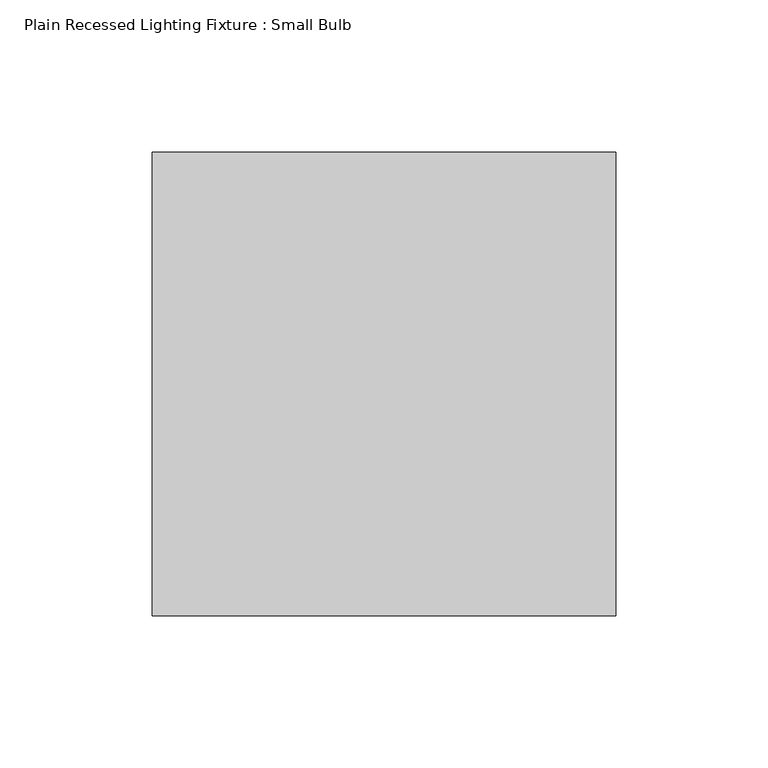
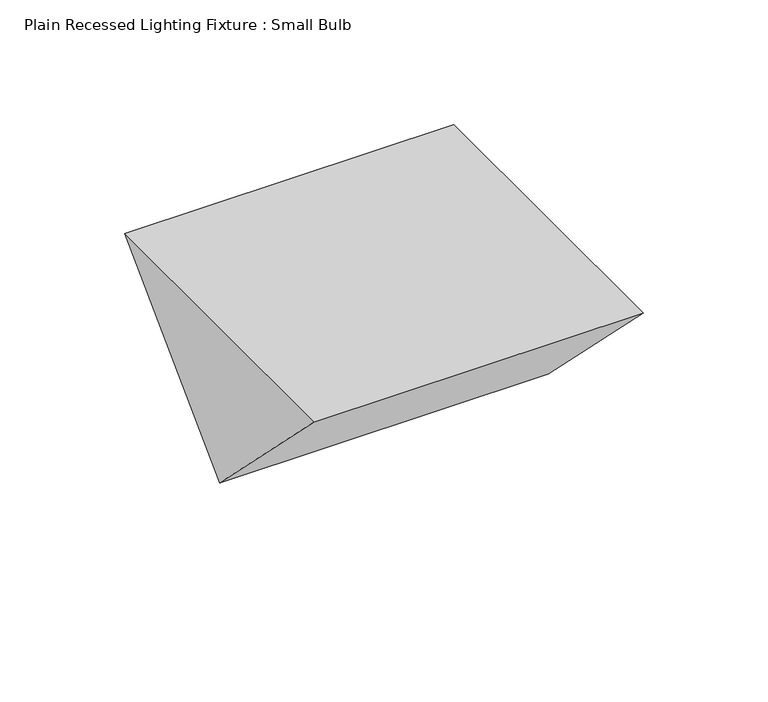
"""IFC4 building model written with IfcOpenShell, lengths in millimetres: light fixture geometry, Plain Recessed Lighting Fixture : Small Bulb."""

from ifc_helpers import new_model, si_unit, frame, origin, place, context, project, spatial, polyline, outline, extrude, source, transform, mapped, element, save


def plain_recessed_lighting_fixture_small_bulb_b229a362(model_context):
    return source(origin(), model_context, "Body", "SweptSolid", [
        extrude(outline(polyline([(-152.4, 0.0), (0.0, 0.0), (-76.2, -76.2), (-152.4, 0.0)])), frame((0.0, 0.0, 0.0), z_axis=(1.0, 0.0, 0.0), x_axis=(0.0, 1.0, 0.0)), (0.0, 0.0, 1.0), 152.4),
    ])


if __name__ == "__main__":
    model = new_model("IFC4")
    model_context = context("Model", 3, world=origin())
    ifc_project = project(units=[si_unit("LENGTHUNIT", "METRE", prefix="MILLI")], contexts=[model_context])
    site = spatial("IfcSite", under=ifc_project)
    building = spatial("IfcBuilding", under=site)
    placement = place(None, origin())
    plain_recessed_lighting_fixture_small_bulb_shape = plain_recessed_lighting_fixture_small_bulb_b229a362(model_context)
    element("IfcLightFixture", 1, ObjectType="Plain Recessed Lighting Fixture : Small Bulb", at=placement, inside=building, context=model_context, shape_type="MappedRepresentation", body=[
        mapped(plain_recessed_lighting_fixture_small_bulb_shape, transform((0.0, 0.0, 0.0), x_axis=(1.0, 0.0, 0.0), y_axis=(0.0, 1.0, 0.0), z_axis=(0.0, 0.0, 1.0))),
    ])
    save(model, "model.ifc")

# Revit data of these elements
# Type "Plain Recessed Lighting Fixture : Small Bulb"
#   Photometric Web File = "2x22UA12.ies"
#   Width = 0' - 6"
#   Wattage = 62 W
#   built-in parameter 1150110 = 1 (stored number, unit not read)
#   built-in parameter 1150109 = 1 (stored number, unit not read)
#   built-in parameter 1150113 = 1 (stored number, unit not read)
#   Tilt Angle = -90.00°
#   Lumens = 5199.94 lm
#   built-in parameter 1114217 = 0.88 (stored number, unit not read)
#   built-in parameter 1150115 = 1 (stored number, unit not read)
#   built-in parameter 1150105 = 413.798 (stored number, unit not read)
#   Length = 0' - 6"
#   built-in parameter 1150112 = 1 (stored number, unit not read)
#   built-in parameter 1150114 = 1 (stored number, unit not read)
#   built-in parameter 1150107 = 4230 (stored number, unit not read)
#   built-in parameter 1150106 = 4.13798 (stored number, unit not read)
#   Emit from Rectangle Width = 0' - 6"
#   Emit from Rectangle Length = 0' - 6"
#   built-in parameter 1150104 = 7.79178 (stored number, unit not read)
#   Depth = 0' - 6"
#   Default Elevation = 4' - 0"
#   Ballast Voltage = 120 V
#   built-in parameter 1114218 = 0.88 (stored number, unit not read)
#   built-in parameter 1150133 = 10 (stored number, unit not read)
#   Apparent Load = 62 VA
#   built-in parameter 1150134 = 8
#   built-in parameter 1150137 = 1
#   Color Filter = 16777215
#   built-in parameter 1140040 [instance default] = 1
#   Load Classification = Lighting - Dwelling Unit
#   Emit Shape Visible in Rendering = no
#   Dimming Lamp Color Temperature Shift = (empty or 0)
#   Assembly Code = ""
